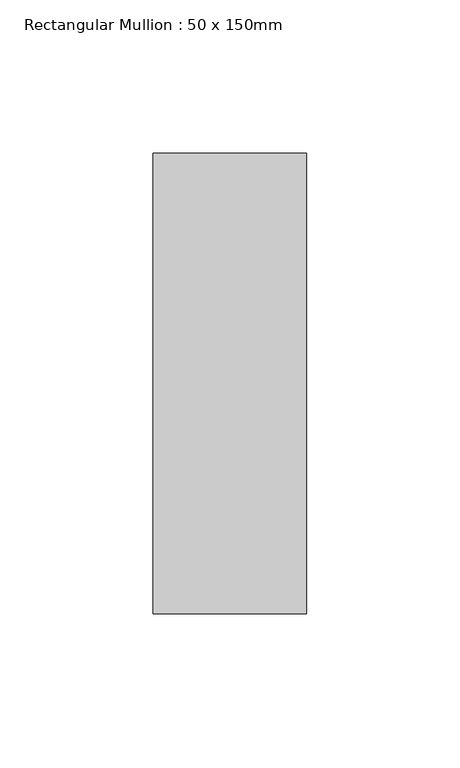
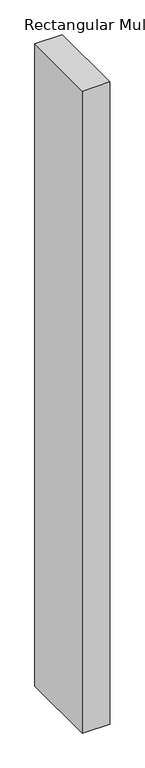
"""IFC4 building model written with IfcOpenShell, lengths in millimetres: member geometry, Rectangular Mullion : 50 x 150mm."""

import ifcopenshell
import ifcopenshell.guid

model = None  # the IFC model being written
_history = None  # IfcOwnerHistory: only IFC2X3 demands one
_inside = {}  # id of a spatial element -> (the spatial element, [elements in it])
_under = {}  # id of a project, library or spatial element -> (it, [spatial elements below it])
_declared = {}  # id of a project -> (the project, [libraries it declares])
_typed = {}  # id of a type object -> (the type object, [elements of that type])
_made_of = {}  # id of a material, layer set ... -> (it, [elements and type objects made of it])


def new_model(schema):
    """Start an empty IFC model of exactly this schema.

    Asked for "IFC4X3", IfcOpenShell would pick the latest addendum, in which some entities
    have other attributes; the version numbers below select the first issue.
    IFC2X3 requires an IfcOwnerHistory on every rooted entity: one is made here for all.
    """
    global model, _history
    if schema == "IFC4X3":
        model = ifcopenshell.file(schema_version=(4, 3, 0, 0))
    else:
        model = ifcopenshell.file(schema=schema)
    _inside.clear()
    _under.clear()
    _declared.clear()
    _typed.clear()
    _made_of.clear()
    _history = None
    if model.schema == "IFC2X3":
        org = make("IfcOrganization", Name="unknown")
        user = make(
            "IfcPersonAndOrganization",
            ThePerson=make("IfcPerson", FamilyName="unknown"),
            TheOrganization=org,
        )
        app = make(
            "IfcApplication",
            ApplicationDeveloper=org,
            Version="unknown",
            ApplicationFullName="unknown",
            ApplicationIdentifier="unknown",
        )
        _history = make(
            "IfcOwnerHistory",
            OwningUser=user,
            OwningApplication=app,
            ChangeAction="ADDED",
            CreationDate=0,
        )
    return model


def make(cls, **values):
    """One entity of the class cls with the attributes given. An attribute that is None is left unset."""
    return model.create_entity(
        cls, **{name: value for name, value in values.items() if value is not None}
    )


def rooted(cls, **values):
    """An entity with a GlobalId (a new one), such as an element, a storey or a relation."""
    return make(cls, GlobalId=ifcopenshell.guid.new(), OwnerHistory=_history, **values)


def si_unit(unit_type, name, prefix=None):
    """IfcSIUnit, for example si_unit("LENGTHUNIT", "METRE", prefix="MILLI")."""
    return make("IfcSIUnit", UnitType=unit_type, Prefix=prefix, Name=name)


def assignment(units):
    """IfcUnitAssignment: the units of a project."""
    return None if units is None else make("IfcUnitAssignment", Units=units)


def point(xyz):
    """IfcCartesianPoint."""
    return None if xyz is None else make("IfcCartesianPoint", Coordinates=xyz)


def direction(xyz):
    """IfcDirection."""
    return None if xyz is None else make("IfcDirection", DirectionRatios=xyz)


def frame(location, z_axis=None, x_axis=None):
    """IfcAxis2Placement3D, a coordinate frame: its origin and axes. An axis left out is left unset."""
    return make(
        "IfcAxis2Placement3D",
        Location=point(location),
        Axis=direction(z_axis),
        RefDirection=direction(x_axis),
    )


def origin():
    """The frame at (0, 0, 0) with its axes left unset."""
    return frame((0.0, 0.0, 0.0))


def place(relative_to, where):
    """IfcLocalPlacement: puts the frame where relative to a parent placement (None: the world)."""
    return make(
        "IfcLocalPlacement", PlacementRelTo=relative_to, RelativePlacement=where
    )


def context(
    kind, dimensions, precision=None, world=None, true_north=None, identifier=None
):
    """IfcGeometricRepresentationContext, for example the 3D "Model" context."""
    return make(
        "IfcGeometricRepresentationContext",
        ContextIdentifier=identifier,
        ContextType=kind,
        CoordinateSpaceDimension=dimensions,
        Precision=precision,
        WorldCoordinateSystem=world,
        TrueNorth=true_north,
    )


def project(units=None, contexts=None):
    """IfcProject with its units and contexts."""
    return rooted(
        "IfcProject",
        Name="project",
        RepresentationContexts=contexts,
        UnitsInContext=assignment(units),
    )


def spatial(cls, under=None, at=None, **own):
    """A site, building, storey or space (cls), placed at a placement, below another one or the project."""
    s = rooted(cls, ObjectPlacement=at, **own)
    if under is not None:
        _under.setdefault(under.id(), (under, []))[1].append(s)
    return s


def polyline(points):
    """IfcPolyline through the points."""
    return make("IfcPolyline", Points=[point(p) for p in points])


def outline(outer, holes=None, kind="AREA"):
    """IfcArbitraryClosedProfileDef: a profile drawn as a closed curve; with holes, ...WithVoids."""
    if holes is None:
        return make("IfcArbitraryClosedProfileDef", ProfileType=kind, OuterCurve=outer)
    return make(
        "IfcArbitraryProfileDefWithVoids",
        ProfileType=kind,
        OuterCurve=outer,
        InnerCurves=holes,
    )


def extrude(swept, where, along, depth):
    """IfcExtrudedAreaSolid: the profile swept, set in the frame where, extruded along a direction by depth."""
    return make(
        "IfcExtrudedAreaSolid",
        SweptArea=swept,
        Position=where,
        ExtrudedDirection=direction(along),
        Depth=depth,
    )


def shape(context_of_items, identifier, shape_type, items):
    """IfcShapeRepresentation: the items that make up one representation, for example the "Body"."""
    return make(
        "IfcShapeRepresentation",
        ContextOfItems=context_of_items,
        RepresentationIdentifier=identifier,
        RepresentationType=shape_type,
        Items=items,
    )


def source(mapping_origin, context_of_items, identifier, shape_type, items):
    """IfcRepresentationMap: a shape defined once, which mapped items show again and again."""
    return make(
        "IfcRepresentationMap",
        MappingOrigin=mapping_origin,
        MappedRepresentation=shape(context_of_items, identifier, shape_type, items),
    )


def transform(
    local_origin,
    x_axis=None,
    y_axis=None,
    z_axis=None,
    scale=None,
    scale2=None,
    scale3=None,
    uniform=True,
):
    """IfcCartesianTransformationOperator3D, or its non-uniform kind. x_axis, y_axis, z_axis: its Axis1, 2, 3."""
    if uniform:
        return make(
            "IfcCartesianTransformationOperator3D",
            Axis1=direction(x_axis),
            Axis2=direction(y_axis),
            LocalOrigin=point(local_origin),
            Scale=scale,
            Axis3=direction(z_axis),
        )
    return make(
        "IfcCartesianTransformationOperator3DnonUniform",
        Axis1=direction(x_axis),
        Axis2=direction(y_axis),
        LocalOrigin=point(local_origin),
        Scale=scale,
        Axis3=direction(z_axis),
        Scale2=scale2,
        Scale3=scale3,
    )


def mapped(mapping_source, mapping_target):
    """IfcMappedItem: shows the shape of a source again, moved by a transform."""
    return make(
        "IfcMappedItem", MappingSource=mapping_source, MappingTarget=mapping_target
    )


def made_of(thing, what):
    """Note that an element or type object is made of a material, layer set ...; save() writes the relation."""
    if what is not None:
        _made_of.setdefault(what.id(), (what, []))[1].append(thing)
    return thing


def element(
    cls,
    number,
    at=None,
    inside=None,
    cuts=None,
    type_object=None,
    material=None,
    context=None,
    identifier="Body",
    shape_type=None,
    held_by="IfcProductDefinitionShape",
    body=None,
    shapes=None,
    **own,
):
    """One element of the class cls, such as IfcWall. Its Tag is "e" and its number.

    at: its placement. inside: the storey or other place that contains it. cuts: it is an
    opening in that element (IfcRelVoidsElement). A single representation is given by context,
    identifier, shape_type and body (its items); several are given by shapes. held_by: the class
    of the entity that holds the representations. save() writes the other relations.
    """
    e = rooted(cls, Tag="e%d" % number, ObjectPlacement=at, **own)
    if body is not None:
        shapes = [shape(context, identifier, shape_type, body)]
    if shapes is not None:
        e.Representation = make(held_by, Representations=shapes)
    if inside is not None:
        _inside.setdefault(inside.id(), (inside, []))[1].append(e)
    if cuts is not None:
        rooted(
            "IfcRelVoidsElement", RelatingBuildingElement=cuts, RelatedOpeningElement=e
        )
    if type_object is not None:
        _typed.setdefault(type_object.id(), (type_object, []))[1].append(e)
    return made_of(e, material)


def aggregate(whole, parts):
    """IfcRelAggregates: a whole, such as a stair, and the parts it consists of."""
    return rooted("IfcRelAggregates", RelatingObject=whole, RelatedObjects=parts)


def save(model, path):
    """Write the relations noted so far, then the file.

    IfcRelAggregates (storeys below a building ...), IfcRelContainedInSpatialStructure (elements
    in a storey), IfcRelDefinesByType, IfcRelAssociatesMaterial and IfcRelDeclares: one each for
    every whole, place, type object, material and project.
    """
    for whole, parts in _under.values():
        aggregate(whole, parts)
    for where, things in _inside.values():
        rooted(
            "IfcRelContainedInSpatialStructure",
            RelatedElements=things,
            RelatingStructure=where,
        )
    for kind, things in _typed.values():
        rooted("IfcRelDefinesByType", RelatedObjects=things, RelatingType=kind)
    for what, things in _made_of.values():
        rooted("IfcRelAssociatesMaterial", RelatedObjects=things, RelatingMaterial=what)
    for by, libraries in _declared.values():
        rooted("IfcRelDeclares", RelatingContext=by, RelatedDefinitions=libraries)
    model.write(path)


def rectangular_mullion_50_x_150mm_31ac4966(model_context):
    return source(origin(), model_context, "Body", "SweptSolid", [
        extrude(outline(polyline([(0.0, 75.0), (0.0, -75.0), (-50.0, -75.0), (-50.0, 75.0), (0.0, 75.0)])), frame((0.0, 0.0, -1241.1082713), z_axis=(0.0, 0.0, 1.0), x_axis=(1.0, 0.0, 0.0)), (0.0, 0.0, 1.0), 1241.1082713),
    ])


if __name__ == "__main__":
    model = new_model("IFC4")
    model_context = context("Model", 3, world=origin())
    ifc_project = project(units=[si_unit("LENGTHUNIT", "METRE", prefix="MILLI")], contexts=[model_context])
    site = spatial("IfcSite", under=ifc_project)
    building = spatial("IfcBuilding", under=site)
    placement = place(None, origin())
    rectangular_mullion_50_x_150mm_shape = rectangular_mullion_50_x_150mm_31ac4966(model_context)
    element("IfcMember", 1, ObjectType="Rectangular Mullion : 50 x 150mm", at=placement, inside=building, context=model_context, shape_type="MappedRepresentation", body=[
        mapped(rectangular_mullion_50_x_150mm_shape, transform((0.0, 0.0, 0.0), x_axis=(1.0, 0.0, 0.0), y_axis=(0.0, 1.0, 0.0), z_axis=(0.0, 0.0, 1.0))),
    ])
    save(model, "model.ifc")

# Revit data of these elements
# Type "Rectangular Mullion : 50 x 150mm"
#   built-in parameter 1007304 = 0.492126 (stored number, unit not read)
#   built-in parameter 1007301 = 0.082021 (stored number, unit not read)
#   built-in parameter 1007300 = 0.082021 (stored number, unit not read)
# Element 1 (IfcMember, "Rectangular Mullion : 50 x 150mm")
#   Materials on its faces: "Aluminium"
# Materials
#   "Aluminium": class "Metal", colour RGB 247 247 247, transparency 0, Description = "Aluminium 6061", Cost = 0
